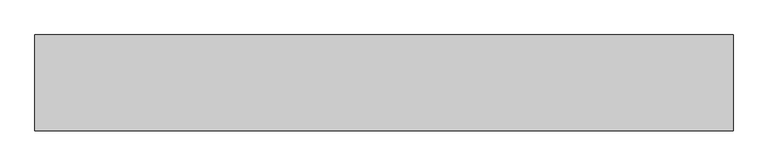
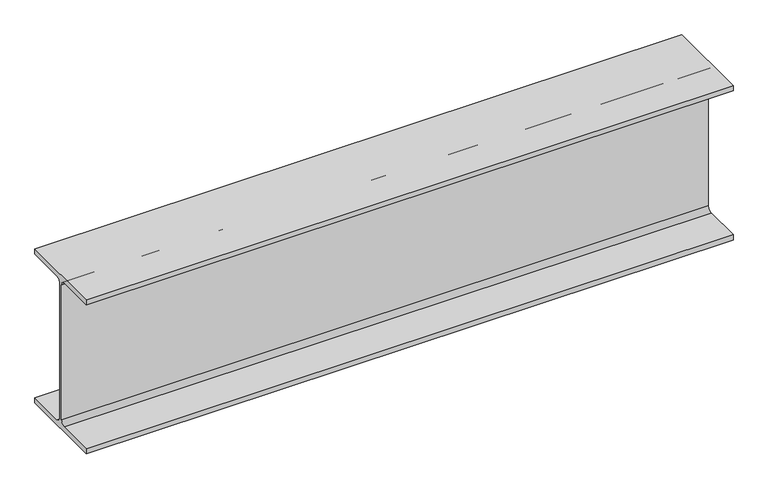
"""IFC4 building model written with IfcOpenShell, lengths in millimetres: beam geometry, Old_Steel Beam_H-KSD3502 : H_SB_ASB_H-194×150x6x9."""

import ifcopenshell
import ifcopenshell.guid

model = None  # the IFC model being written
_history = None  # IfcOwnerHistory: only IFC2X3 demands one
_inside = {}  # id of a spatial element -> (the spatial element, [elements in it])
_under = {}  # id of a project, library or spatial element -> (it, [spatial elements below it])
_declared = {}  # id of a project -> (the project, [libraries it declares])
_typed = {}  # id of a type object -> (the type object, [elements of that type])
_made_of = {}  # id of a material, layer set ... -> (it, [elements and type objects made of it])


def new_model(schema):
    """Start an empty IFC model of exactly this schema.

    Asked for "IFC4X3", IfcOpenShell would pick the latest addendum, in which some entities
    have other attributes; the version numbers below select the first issue.
    IFC2X3 requires an IfcOwnerHistory on every rooted entity: one is made here for all.
    """
    global model, _history
    if schema == "IFC4X3":
        model = ifcopenshell.file(schema_version=(4, 3, 0, 0))
    else:
        model = ifcopenshell.file(schema=schema)
    _inside.clear()
    _under.clear()
    _declared.clear()
    _typed.clear()
    _made_of.clear()
    _history = None
    if model.schema == "IFC2X3":
        org = make("IfcOrganization", Name="unknown")
        user = make(
            "IfcPersonAndOrganization",
            ThePerson=make("IfcPerson", FamilyName="unknown"),
            TheOrganization=org,
        )
        app = make(
            "IfcApplication",
            ApplicationDeveloper=org,
            Version="unknown",
            ApplicationFullName="unknown",
            ApplicationIdentifier="unknown",
        )
        _history = make(
            "IfcOwnerHistory",
            OwningUser=user,
            OwningApplication=app,
            ChangeAction="ADDED",
            CreationDate=0,
        )
    return model


def make(cls, **values):
    """One entity of the class cls with the attributes given. An attribute that is None is left unset."""
    return model.create_entity(
        cls, **{name: value for name, value in values.items() if value is not None}
    )


def rooted(cls, **values):
    """An entity with a GlobalId (a new one), such as an element, a storey or a relation."""
    return make(cls, GlobalId=ifcopenshell.guid.new(), OwnerHistory=_history, **values)


def si_unit(unit_type, name, prefix=None):
    """IfcSIUnit, for example si_unit("LENGTHUNIT", "METRE", prefix="MILLI")."""
    return make("IfcSIUnit", UnitType=unit_type, Prefix=prefix, Name=name)


def assignment(units):
    """IfcUnitAssignment: the units of a project."""
    return None if units is None else make("IfcUnitAssignment", Units=units)


def point(xyz):
    """IfcCartesianPoint."""
    return None if xyz is None else make("IfcCartesianPoint", Coordinates=xyz)


def direction(xyz):
    """IfcDirection."""
    return None if xyz is None else make("IfcDirection", DirectionRatios=xyz)


def frame(location, z_axis=None, x_axis=None):
    """IfcAxis2Placement3D, a coordinate frame: its origin and axes. An axis left out is left unset."""
    return make(
        "IfcAxis2Placement3D",
        Location=point(location),
        Axis=direction(z_axis),
        RefDirection=direction(x_axis),
    )


def frame_2d(location, x_axis=None):
    """IfcAxis2Placement2D, a coordinate frame in the plane: its origin and x axis."""
    return make(
        "IfcAxis2Placement2D", Location=point(location), RefDirection=direction(x_axis)
    )


def origin():
    """The frame at (0, 0, 0) with its axes left unset."""
    return frame((0.0, 0.0, 0.0))


def place(relative_to, where):
    """IfcLocalPlacement: puts the frame where relative to a parent placement (None: the world)."""
    return make(
        "IfcLocalPlacement", PlacementRelTo=relative_to, RelativePlacement=where
    )


def context(
    kind, dimensions, precision=None, world=None, true_north=None, identifier=None
):
    """IfcGeometricRepresentationContext, for example the 3D "Model" context."""
    return make(
        "IfcGeometricRepresentationContext",
        ContextIdentifier=identifier,
        ContextType=kind,
        CoordinateSpaceDimension=dimensions,
        Precision=precision,
        WorldCoordinateSystem=world,
        TrueNorth=true_north,
    )


def project(units=None, contexts=None):
    """IfcProject with its units and contexts."""
    return rooted(
        "IfcProject",
        Name="project",
        RepresentationContexts=contexts,
        UnitsInContext=assignment(units),
    )


def spatial(cls, under=None, at=None, **own):
    """A site, building, storey or space (cls), placed at a placement, below another one or the project."""
    s = rooted(cls, ObjectPlacement=at, **own)
    if under is not None:
        _under.setdefault(under.id(), (under, []))[1].append(s)
    return s


def polyline(points):
    """IfcPolyline through the points."""
    return make("IfcPolyline", Points=[point(p) for p in points])


def circle_curve(where, radius):
    """IfcCircle in the frame where."""
    return make("IfcCircle", Position=where, Radius=radius)


def trimmed(basis, trim1, trim2, sense, master):
    """IfcTrimmedCurve: the piece of a basis curve between two trims."""
    return make(
        "IfcTrimmedCurve",
        BasisCurve=basis,
        Trim1=trim1,
        Trim2=trim2,
        SenseAgreement=sense,
        MasterRepresentation=master,
    )


def segment(curve, same_sense, transition):
    """IfcCompositeCurveSegment."""
    return make(
        "IfcCompositeCurveSegment",
        Transition=transition,
        SameSense=same_sense,
        ParentCurve=curve,
    )


def composite_curve(segments, self_intersect=None):
    """IfcCompositeCurve: segments joined end to end."""
    return make("IfcCompositeCurve", Segments=segments, SelfIntersect=self_intersect)


def outline(outer, holes=None, kind="AREA"):
    """IfcArbitraryClosedProfileDef: a profile drawn as a closed curve; with holes, ...WithVoids."""
    if holes is None:
        return make("IfcArbitraryClosedProfileDef", ProfileType=kind, OuterCurve=outer)
    return make(
        "IfcArbitraryProfileDefWithVoids",
        ProfileType=kind,
        OuterCurve=outer,
        InnerCurves=holes,
    )


def extrude(swept, where, along, depth):
    """IfcExtrudedAreaSolid: the profile swept, set in the frame where, extruded along a direction by depth."""
    return make(
        "IfcExtrudedAreaSolid",
        SweptArea=swept,
        Position=where,
        ExtrudedDirection=direction(along),
        Depth=depth,
    )


def shape(context_of_items, identifier, shape_type, items):
    """IfcShapeRepresentation: the items that make up one representation, for example the "Body"."""
    return make(
        "IfcShapeRepresentation",
        ContextOfItems=context_of_items,
        RepresentationIdentifier=identifier,
        RepresentationType=shape_type,
        Items=items,
    )


def source(mapping_origin, context_of_items, identifier, shape_type, items):
    """IfcRepresentationMap: a shape defined once, which mapped items show again and again."""
    return make(
        "IfcRepresentationMap",
        MappingOrigin=mapping_origin,
        MappedRepresentation=shape(context_of_items, identifier, shape_type, items),
    )


def transform(
    local_origin,
    x_axis=None,
    y_axis=None,
    z_axis=None,
    scale=None,
    scale2=None,
    scale3=None,
    uniform=True,
):
    """IfcCartesianTransformationOperator3D, or its non-uniform kind. x_axis, y_axis, z_axis: its Axis1, 2, 3."""
    if uniform:
        return make(
            "IfcCartesianTransformationOperator3D",
            Axis1=direction(x_axis),
            Axis2=direction(y_axis),
            LocalOrigin=point(local_origin),
            Scale=scale,
            Axis3=direction(z_axis),
        )
    return make(
        "IfcCartesianTransformationOperator3DnonUniform",
        Axis1=direction(x_axis),
        Axis2=direction(y_axis),
        LocalOrigin=point(local_origin),
        Scale=scale,
        Axis3=direction(z_axis),
        Scale2=scale2,
        Scale3=scale3,
    )


def mapped(mapping_source, mapping_target):
    """IfcMappedItem: shows the shape of a source again, moved by a transform."""
    return make(
        "IfcMappedItem", MappingSource=mapping_source, MappingTarget=mapping_target
    )


def made_of(thing, what):
    """Note that an element or type object is made of a material, layer set ...; save() writes the relation."""
    if what is not None:
        _made_of.setdefault(what.id(), (what, []))[1].append(thing)
    return thing


def element(
    cls,
    number,
    at=None,
    inside=None,
    cuts=None,
    type_object=None,
    material=None,
    context=None,
    identifier="Body",
    shape_type=None,
    held_by="IfcProductDefinitionShape",
    body=None,
    shapes=None,
    **own,
):
    """One element of the class cls, such as IfcWall. Its Tag is "e" and its number.

    at: its placement. inside: the storey or other place that contains it. cuts: it is an
    opening in that element (IfcRelVoidsElement). A single representation is given by context,
    identifier, shape_type and body (its items); several are given by shapes. held_by: the class
    of the entity that holds the representations. save() writes the other relations.
    """
    e = rooted(cls, Tag="e%d" % number, ObjectPlacement=at, **own)
    if body is not None:
        shapes = [shape(context, identifier, shape_type, body)]
    if shapes is not None:
        e.Representation = make(held_by, Representations=shapes)
    if inside is not None:
        _inside.setdefault(inside.id(), (inside, []))[1].append(e)
    if cuts is not None:
        rooted(
            "IfcRelVoidsElement", RelatingBuildingElement=cuts, RelatedOpeningElement=e
        )
    if type_object is not None:
        _typed.setdefault(type_object.id(), (type_object, []))[1].append(e)
    return made_of(e, material)


def aggregate(whole, parts):
    """IfcRelAggregates: a whole, such as a stair, and the parts it consists of."""
    return rooted("IfcRelAggregates", RelatingObject=whole, RelatedObjects=parts)


def save(model, path):
    """Write the relations noted so far, then the file.

    IfcRelAggregates (storeys below a building ...), IfcRelContainedInSpatialStructure (elements
    in a storey), IfcRelDefinesByType, IfcRelAssociatesMaterial and IfcRelDeclares: one each for
    every whole, place, type object, material and project.
    """
    for whole, parts in _under.values():
        aggregate(whole, parts)
    for where, things in _inside.values():
        rooted(
            "IfcRelContainedInSpatialStructure",
            RelatedElements=things,
            RelatingStructure=where,
        )
    for kind, things in _typed.values():
        rooted("IfcRelDefinesByType", RelatedObjects=things, RelatingType=kind)
    for what, things in _made_of.values():
        rooted("IfcRelAssociatesMaterial", RelatedObjects=things, RelatingMaterial=what)
    for by, libraries in _declared.values():
        rooted("IfcRelDeclares", RelatingContext=by, RelatedDefinitions=libraries)
    model.write(path)


def beam_8feac67b(model_context):
    return source(origin(), model_context, "Body", "SweptSolid", [
        extrude(outline(composite_curve([segment(polyline([(82.5, -141.5), (82.5, -151.7), (-82.5, -151.7), (-82.5, -141.5), (-11.9, -141.5)]), True, "CONTINUOUS"), segment(trimmed(circle_curve(frame_2d((-11.9, -132.6)), 8.9), [point((-11.9, -141.5))], [point((-3.0, -132.6))], True, "CARTESIAN"), True, "CONTINUOUS"), segment(polyline([(-3.0, -132.6), (-3.0, 132.6)]), True, "CONTINUOUS"), segment(trimmed(circle_curve(frame_2d((-11.9, 132.6)), 8.9), [point((-3.0, 132.6))], [point((-11.9, 141.5))], True, "CARTESIAN"), True, "CONTINUOUS"), segment(polyline([(-11.9, 141.5), (-82.5, 141.5), (-82.5, 151.7), (82.5, 151.7), (82.5, 141.5), (11.9, 141.5)]), True, "CONTINUOUS"), segment(trimmed(circle_curve(frame_2d((11.9, 132.6)), 8.9), [point((11.9, 141.5))], [point((3.0, 132.6))], True, "CARTESIAN"), True, "CONTINUOUS"), segment(polyline([(3.0, 132.6), (3.0, -132.6)]), True, "CONTINUOUS"), segment(trimmed(circle_curve(frame_2d((11.9, -132.6)), 8.9), [point((3.0, -132.6))], [point((11.9, -141.5))], True, "CARTESIAN"), True, "CONTINUOUS"), segment(polyline([(11.9, -141.5), (82.5, -141.5)]), True, "CONTINUOUS")], self_intersect=False)), frame((-601.6366265, 0.0, 0.0), z_axis=(1.0, 0.0, 0.0), x_axis=(0.0, 1.0, 0.0)), (0.0, 0.0, 1.0), 1203.2732531),
    ])


if __name__ == "__main__":
    model = new_model("IFC4")
    model_context = context("Model", 3, world=origin())
    ifc_project = project(units=[si_unit("LENGTHUNIT", "METRE", prefix="MILLI")], contexts=[model_context])
    site = spatial("IfcSite", under=ifc_project)
    building = spatial("IfcBuilding", under=site)
    placement = place(None, origin())
    beam_shape = beam_8feac67b(model_context)
    element("IfcBeam", 1, ObjectType="Old_Steel Beam_H-KSD3502 : H_SB_ASB_H-194×150x6x9", at=placement, inside=building, context=model_context, shape_type="MappedRepresentation", body=[
        mapped(beam_shape, transform((0.0, 0.0, 0.0), x_axis=(1.0, 0.0, 0.0), y_axis=(0.0, 1.0, 0.0), z_axis=(0.0, 0.0, 1.0))),
    ])
    save(model, "model.ifc")

# Revit data of these elements
# Type "Old_Steel Beam_H-KSD3502 : H_SB_ASB_H-194×150x6x9"
#   Width = 15.0 cm
#   Web Thickness = 0.6 cm
#   Web Fillet = 1.3 cm
#   Warping Constant = 43316.0 cm⁶
#   Torsional Moment of Inertia = 8.622 cm⁴
#   Torsional Modulus = 1.0 cm³
#   Section Area = 39.01 cm²
#   Plastic Modulus weak axis = 104.0 cm³
#   Plastic Modulus strong axis = 309.0 cm³
#   Perimeter = 0.95 m²/m
#   Nominal Weight = 30.60 kgf/m
#   Moment of Inertia weak axis = 507.00 cm⁴
#   Moment of Inertia strong axis = 2690.00 cm⁴
#   Height = 19.4 cm
#   Flange Thickness = 0.9 cm
#   Elastic Modulus weak axis = 67.6 cm³
#   Elastic Modulus strong axis = 277.0 cm³
#   Centroid Vertical = 9.7 cm
#   Centroid Horizontal = 7.5 cm
#   Length [instance default] = 1.5240 m
#   Structural Material [instance default] = Steel, 45-345
#   Assembly Code = ""
# Element 1 (IfcBeam, "Old_Steel Beam_H-KSD3502 : H_SB_ASB_H-194×150x6x9")
#   Structural Material = none
# Materials
#   "Steel, 45-345": class "Metal", colour RGB 189 187 185, transparency 0, Description = "Steel 345 MPa", Cost = 0
